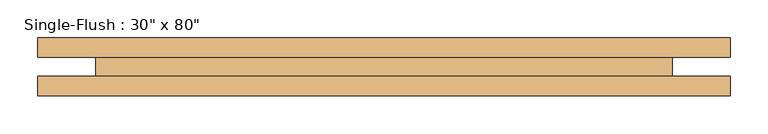
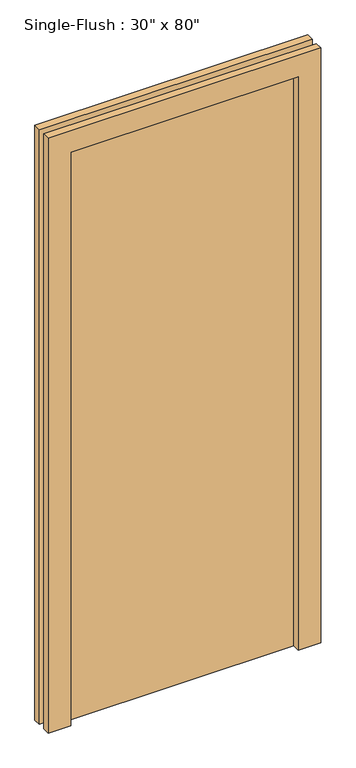
"""IFC4 building model written with IfcOpenShell, lengths in millimetres: door geometry."""

from ifc_helpers import new_model, si_unit, frame, origin, origin_with_axes, place, context, project, spatial, polyline, outline, extrude, source, transform, mapped, element, save


def door_cef5613e(model_context):
    return source(origin(), model_context, "Body", "SweptSolid", [
        extrude(outline(polyline([(2108.2, -457.2), (0.0, -457.2), (0.0, -381.0), (2032.0, -381.0), (2032.0, 381.0), (0.0, 381.0), (0.0, 457.2), (2108.2, 457.2), (2108.2, -457.2)])), frame((0.0, -38.1, 0.0), z_axis=(0.0, 1.0, 0.0), x_axis=(0.0, 0.0, 1.0)), (0.0, 0.0, 1.0), 25.4),
        extrude(outline(polyline([(2108.2, 457.2), (2108.2, -457.2), (0.0, -457.2), (0.0, -381.0), (2032.0, -381.0), (2032.0, 381.0), (0.0, 381.0), (0.0, 457.2), (2108.2, 457.2)])), frame((0.0, 12.7, 0.0), z_axis=(0.0, 1.0, 0.0), x_axis=(0.0, 0.0, 1.0)), (0.0, 0.0, 1.0), 25.4),
        extrude(outline(polyline([(381.0, 38.1), (381.0, -12.7), (-381.0, -12.7), (-381.0, 38.1), (381.0, 38.1)])), origin_with_axes(), (0.0, 0.0, 1.0), 2032.0),
    ])


if __name__ == "__main__":
    model = new_model("IFC4")
    model_context = context("Model", 3, world=origin())
    ifc_project = project(units=[si_unit("LENGTHUNIT", "METRE", prefix="MILLI")], contexts=[model_context])
    site = spatial("IfcSite", under=ifc_project)
    building = spatial("IfcBuilding", under=site)
    placement = place(None, origin())
    door_shape = door_cef5613e(model_context)
    element("IfcDoor", 1, ObjectType="Single-Flush : 30\" x 80\"", at=placement, inside=building, context=model_context, shape_type="MappedRepresentation", body=[
        mapped(door_shape, transform((0.0, 0.0, 0.0), x_axis=(1.0, 0.0, 0.0), y_axis=(0.0, 1.0, 0.0), z_axis=(0.0, 0.0, 1.0))),
    ])
    save(model, "model.ifc")

# Revit data of these elements
# Type "Single-Flush : 30\" x 80\""
#   Type Mark = "5"
#   Construction Type Id = "MDOOR"
#   Assembly Code = "C1020"
#   Analytic Construction = "Metal"
#   Thickness = 0' - 2"
#   Heat Transfer Coefficient (U) = 0.651978 BTU/(h·ft²·°F)
#   Height = 6' - 8"
#   Trim Projection Ext = 0' - 1"
#   Trim Projection Int = 0' - 1"
#   Trim Width = 0' - 3"
#   Width = 2' - 6"
#   Define Thermal Properties by = 1
#   Define Thermal Properties by = 1
#   Door Material = Door - Panel
#   Frame Material = Door - Frame
#   Visual Light Transmittance = 0
#   Solar Heat Gain Coefficient = 0
#   Function = (empty or 0)
#   Wall Closure = (empty or 0)
# Element 1 (IfcDoor, "Single-Flush : 30\" x 80\"")
#   Materials on its faces: "Door - Frame", "Door - Panel"
# Materials
#   "Door - Panel": class "Wood", colour RGB 210 159 95, transparency 0, Cost = 0
#   "Door - Frame": class "Miscellaneous", colour RGB 118 70 51, transparency 0, Cost = 0
